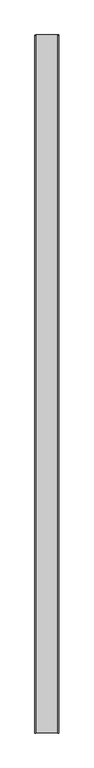
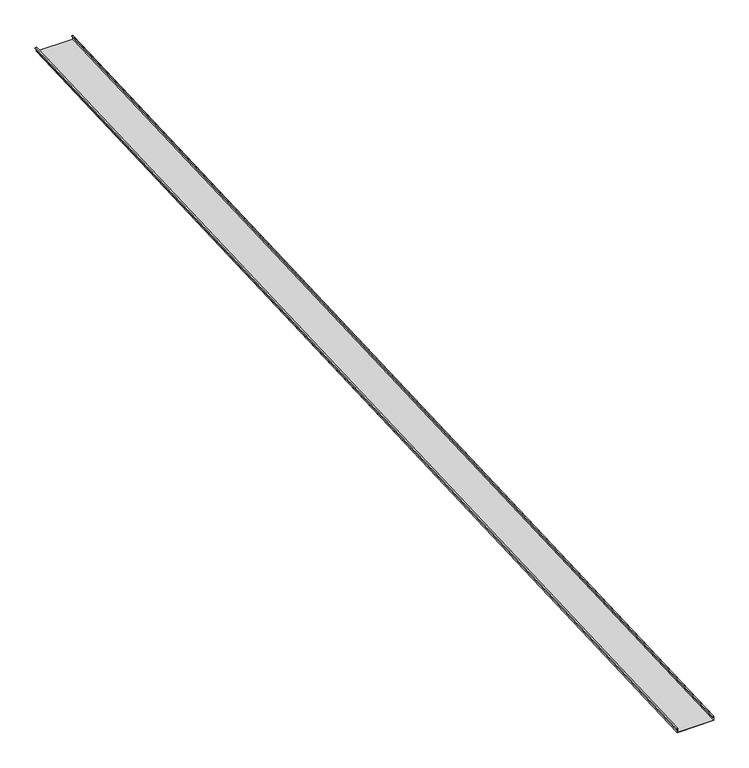
"""IFC4 building model written with IfcOpenShell, lengths in millimetres: proxy geometry, Generic Models 2:Generic Models 2:310765:Generic Models 2:310765 : Generic Models 2:Generic Models 2:310765:34 : Generic Models 2:Generic Models 2:310765:Generic Models 2:310765 : Generic Models 2:Generic Models 2:310765:300385."""

import ifcopenshell
import ifcopenshell.guid

model = None  # the IFC model being written
_history = None  # IfcOwnerHistory: only IFC2X3 demands one
_inside = {}  # id of a spatial element -> (the spatial element, [elements in it])
_under = {}  # id of a project, library or spatial element -> (it, [spatial elements below it])
_declared = {}  # id of a project -> (the project, [libraries it declares])
_typed = {}  # id of a type object -> (the type object, [elements of that type])
_made_of = {}  # id of a material, layer set ... -> (it, [elements and type objects made of it])


def new_model(schema):
    """Start an empty IFC model of exactly this schema.

    Asked for "IFC4X3", IfcOpenShell would pick the latest addendum, in which some entities
    have other attributes; the version numbers below select the first issue.
    IFC2X3 requires an IfcOwnerHistory on every rooted entity: one is made here for all.
    """
    global model, _history
    if schema == "IFC4X3":
        model = ifcopenshell.file(schema_version=(4, 3, 0, 0))
    else:
        model = ifcopenshell.file(schema=schema)
    _inside.clear()
    _under.clear()
    _declared.clear()
    _typed.clear()
    _made_of.clear()
    _history = None
    if model.schema == "IFC2X3":
        org = make("IfcOrganization", Name="unknown")
        user = make(
            "IfcPersonAndOrganization",
            ThePerson=make("IfcPerson", FamilyName="unknown"),
            TheOrganization=org,
        )
        app = make(
            "IfcApplication",
            ApplicationDeveloper=org,
            Version="unknown",
            ApplicationFullName="unknown",
            ApplicationIdentifier="unknown",
        )
        _history = make(
            "IfcOwnerHistory",
            OwningUser=user,
            OwningApplication=app,
            ChangeAction="ADDED",
            CreationDate=0,
        )
    return model


def make(cls, **values):
    """One entity of the class cls with the attributes given. An attribute that is None is left unset."""
    return model.create_entity(
        cls, **{name: value for name, value in values.items() if value is not None}
    )


def rooted(cls, **values):
    """An entity with a GlobalId (a new one), such as an element, a storey or a relation."""
    return make(cls, GlobalId=ifcopenshell.guid.new(), OwnerHistory=_history, **values)


def si_unit(unit_type, name, prefix=None):
    """IfcSIUnit, for example si_unit("LENGTHUNIT", "METRE", prefix="MILLI")."""
    return make("IfcSIUnit", UnitType=unit_type, Prefix=prefix, Name=name)


def assignment(units):
    """IfcUnitAssignment: the units of a project."""
    return None if units is None else make("IfcUnitAssignment", Units=units)


def point(xyz):
    """IfcCartesianPoint."""
    return None if xyz is None else make("IfcCartesianPoint", Coordinates=xyz)


def direction(xyz):
    """IfcDirection."""
    return None if xyz is None else make("IfcDirection", DirectionRatios=xyz)


def frame(location, z_axis=None, x_axis=None):
    """IfcAxis2Placement3D, a coordinate frame: its origin and axes. An axis left out is left unset."""
    return make(
        "IfcAxis2Placement3D",
        Location=point(location),
        Axis=direction(z_axis),
        RefDirection=direction(x_axis),
    )


def origin():
    """The frame at (0, 0, 0) with its axes left unset."""
    return frame((0.0, 0.0, 0.0))


def place(relative_to, where):
    """IfcLocalPlacement: puts the frame where relative to a parent placement (None: the world)."""
    return make(
        "IfcLocalPlacement", PlacementRelTo=relative_to, RelativePlacement=where
    )


def context(
    kind, dimensions, precision=None, world=None, true_north=None, identifier=None
):
    """IfcGeometricRepresentationContext, for example the 3D "Model" context."""
    return make(
        "IfcGeometricRepresentationContext",
        ContextIdentifier=identifier,
        ContextType=kind,
        CoordinateSpaceDimension=dimensions,
        Precision=precision,
        WorldCoordinateSystem=world,
        TrueNorth=true_north,
    )


def project(units=None, contexts=None):
    """IfcProject with its units and contexts."""
    return rooted(
        "IfcProject",
        Name="project",
        RepresentationContexts=contexts,
        UnitsInContext=assignment(units),
    )


def spatial(cls, under=None, at=None, **own):
    """A site, building, storey or space (cls), placed at a placement, below another one or the project."""
    s = rooted(cls, ObjectPlacement=at, **own)
    if under is not None:
        _under.setdefault(under.id(), (under, []))[1].append(s)
    return s


def polyline(points):
    """IfcPolyline through the points."""
    return make("IfcPolyline", Points=[point(p) for p in points])


def outline(outer, holes=None, kind="AREA"):
    """IfcArbitraryClosedProfileDef: a profile drawn as a closed curve; with holes, ...WithVoids."""
    if holes is None:
        return make("IfcArbitraryClosedProfileDef", ProfileType=kind, OuterCurve=outer)
    return make(
        "IfcArbitraryProfileDefWithVoids",
        ProfileType=kind,
        OuterCurve=outer,
        InnerCurves=holes,
    )


def extrude(swept, where, along, depth):
    """IfcExtrudedAreaSolid: the profile swept, set in the frame where, extruded along a direction by depth."""
    return make(
        "IfcExtrudedAreaSolid",
        SweptArea=swept,
        Position=where,
        ExtrudedDirection=direction(along),
        Depth=depth,
    )


def shape(context_of_items, identifier, shape_type, items):
    """IfcShapeRepresentation: the items that make up one representation, for example the "Body"."""
    return make(
        "IfcShapeRepresentation",
        ContextOfItems=context_of_items,
        RepresentationIdentifier=identifier,
        RepresentationType=shape_type,
        Items=items,
    )


def source(mapping_origin, context_of_items, identifier, shape_type, items):
    """IfcRepresentationMap: a shape defined once, which mapped items show again and again."""
    return make(
        "IfcRepresentationMap",
        MappingOrigin=mapping_origin,
        MappedRepresentation=shape(context_of_items, identifier, shape_type, items),
    )


def transform(
    local_origin,
    x_axis=None,
    y_axis=None,
    z_axis=None,
    scale=None,
    scale2=None,
    scale3=None,
    uniform=True,
):
    """IfcCartesianTransformationOperator3D, or its non-uniform kind. x_axis, y_axis, z_axis: its Axis1, 2, 3."""
    if uniform:
        return make(
            "IfcCartesianTransformationOperator3D",
            Axis1=direction(x_axis),
            Axis2=direction(y_axis),
            LocalOrigin=point(local_origin),
            Scale=scale,
            Axis3=direction(z_axis),
        )
    return make(
        "IfcCartesianTransformationOperator3DnonUniform",
        Axis1=direction(x_axis),
        Axis2=direction(y_axis),
        LocalOrigin=point(local_origin),
        Scale=scale,
        Axis3=direction(z_axis),
        Scale2=scale2,
        Scale3=scale3,
    )


def mapped(mapping_source, mapping_target):
    """IfcMappedItem: shows the shape of a source again, moved by a transform."""
    return make(
        "IfcMappedItem", MappingSource=mapping_source, MappingTarget=mapping_target
    )


def made_of(thing, what):
    """Note that an element or type object is made of a material, layer set ...; save() writes the relation."""
    if what is not None:
        _made_of.setdefault(what.id(), (what, []))[1].append(thing)
    return thing


def element(
    cls,
    number,
    at=None,
    inside=None,
    cuts=None,
    type_object=None,
    material=None,
    context=None,
    identifier="Body",
    shape_type=None,
    held_by="IfcProductDefinitionShape",
    body=None,
    shapes=None,
    **own,
):
    """One element of the class cls, such as IfcWall. Its Tag is "e" and its number.

    at: its placement. inside: the storey or other place that contains it. cuts: it is an
    opening in that element (IfcRelVoidsElement). A single representation is given by context,
    identifier, shape_type and body (its items); several are given by shapes. held_by: the class
    of the entity that holds the representations. save() writes the other relations.
    """
    e = rooted(cls, Tag="e%d" % number, ObjectPlacement=at, **own)
    if body is not None:
        shapes = [shape(context, identifier, shape_type, body)]
    if shapes is not None:
        e.Representation = make(held_by, Representations=shapes)
    if inside is not None:
        _inside.setdefault(inside.id(), (inside, []))[1].append(e)
    if cuts is not None:
        rooted(
            "IfcRelVoidsElement", RelatingBuildingElement=cuts, RelatedOpeningElement=e
        )
    if type_object is not None:
        _typed.setdefault(type_object.id(), (type_object, []))[1].append(e)
    return made_of(e, material)


def aggregate(whole, parts):
    """IfcRelAggregates: a whole, such as a stair, and the parts it consists of."""
    return rooted("IfcRelAggregates", RelatingObject=whole, RelatedObjects=parts)


def save(model, path):
    """Write the relations noted so far, then the file.

    IfcRelAggregates (storeys below a building ...), IfcRelContainedInSpatialStructure (elements
    in a storey), IfcRelDefinesByType, IfcRelAssociatesMaterial and IfcRelDeclares: one each for
    every whole, place, type object, material and project.
    """
    for whole, parts in _under.values():
        aggregate(whole, parts)
    for where, things in _inside.values():
        rooted(
            "IfcRelContainedInSpatialStructure",
            RelatedElements=things,
            RelatingStructure=where,
        )
    for kind, things in _typed.values():
        rooted("IfcRelDefinesByType", RelatedObjects=things, RelatingType=kind)
    for what, things in _made_of.values():
        rooted("IfcRelAssociatesMaterial", RelatedObjects=things, RelatingMaterial=what)
    for by, libraries in _declared.values():
        rooted("IfcRelDeclares", RelatingContext=by, RelatedDefinitions=libraries)
    model.write(path)


def generic_models_59a92c46(model_context):
    return source(origin(), model_context, "Body", "SweptSolid", [
        extrude(outline(polyline([(1.5875, 0.0), (1.5875, 50.8000001), (407.9875, 50.8000001), (407.9875, 1.5875), (396.875, 1.5875), (396.875, 11.1125), (398.4625, 11.1125), (398.4625, 3.175), (406.4, 3.175), (406.4, 49.2125), (3.175, 49.2125), (3.175, -1.5874999), (-14.2875, -1.5874999), (-14.2875, 9.5250001), (-12.7, 9.5250001), (-12.7, 0.0), (1.5875, 0.0)])), frame((592719.1763073, -580685.2753521, 3930.5514309), z_axis=(0.0, 0.9991330730923568, 0.04163054471206784), x_axis=(1.0, 0.0, 0.0)), (0.0, 0.0, 1.0), 12442.9769242),
    ])


if __name__ == "__main__":
    model = new_model("IFC4")
    model_context = context("Model", 3, world=origin())
    ifc_project = project(units=[si_unit("LENGTHUNIT", "METRE", prefix="MILLI")], contexts=[model_context])
    site = spatial("IfcSite", under=ifc_project)
    building = spatial("IfcBuilding", under=site)
    placement = place(None, origin())
    generic_models_shape = generic_models_59a92c46(model_context)
    element("IfcBuildingElementProxy", 1, Name="Generic Models 2:Generic Models 2:310765:Generic Models 2:310765 : Generic Models 2:Generic Models 2:310765:34 : Generic Models 2:Generic Models 2:310765:Generic Models 2:310765 : Generic Models 2:Generic Models 2:310765:300385", ObjectType="Generic Models 2:Generic Models 2:310765:Generic Models 2:310765 : Generic Models 2:Generic Models 2:310765:34 : Generic Models 2:Generic Models 2:310765:Generic Models 2:310765 : Generic Models 2:Generic Models 2:310765:300385", at=placement, inside=building, context=model_context, shape_type="MappedRepresentation", body=[
        mapped(generic_models_shape, transform((0.0, 0.0, 0.0), x_axis=(1.0, 0.0, 0.0), y_axis=(0.0, 1.0, 0.0), z_axis=(0.0, 0.0, 1.0))),
    ])
    save(model, "model.ifc")

# Revit data of these elements
# Type "Generic Models 2:Generic Models 2:310765:Generic Models 2:310765 : Generic Models 2:Generic Models 2:310765:34 : Generic Models 2:Generic Models 2:310765:Generic Models 2:310765 : Generic Models 2:Generic Models 2:310765:300385"
#   NameOverride = "Generic Models 2:Generic Models 2:310765:Generic Models 2:310765 : Generic Models 2:Generic Models 2:310765:300385"
#   ObjectTypeOverride = "Generic Models 2:310765 : Generic Models 2:Generic Models 2:310765"
#   Reference = "Generic Models 2"
#   Tag = "300385"
# Element 1 (IfcBuildingElementProxy, "Generic Models 2:Generic Models 2:310765:Generic Models 2:310765 : Generic Models 2:Generic Models 2:310765:34 : Generic Models 2:Generic Models 2:310765:Generic Models 2:310765 : Generic Models 2:Generic Models 2:310765:300385")
#   Materials on its faces: "STRUCTURAL STANDING SEAM SHEET METAL ROOFING - BATTENLOK - COLOR T.B.D."
# Materials
#   "STRUCTURAL STANDING SEAM SHEET METAL ROOFING - BATTENLOK - COLOR T.B.D.": class "Generic", colour RGB 120 120 120, transparency 0, Cost = 0
